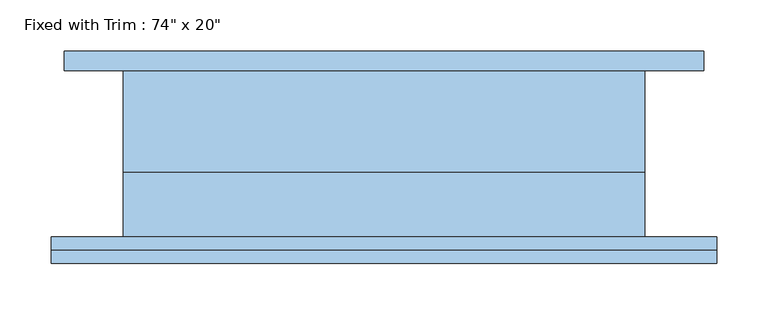
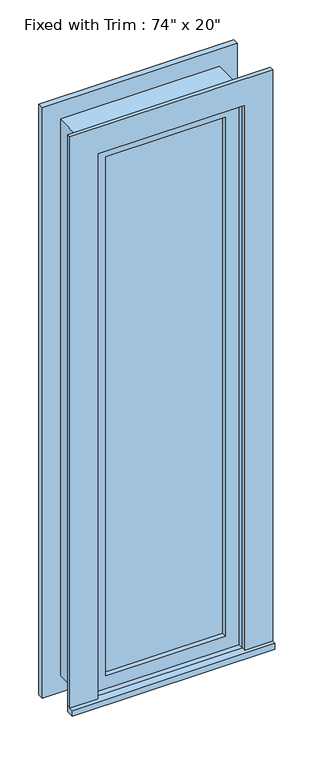
"""IFC4 building model written with IfcOpenShell, lengths in millimetres: window geometry."""

from ifc_helpers import new_model, si_unit, frame, origin, place, context, project, spatial, polyline, outline, extrude, source, transform, mapped, element, save


def window_f2480f1b(model_context):
    return source(origin(), model_context, "Body", "SweptSolid", [
        extrude(outline(polyline([(-361.95, -106.3625), (-361.95, -80.9625), (285.75, -80.9625), (285.75, -106.3625), (-361.95, -106.3625)])), frame((0.0, 0.0, 914.4), z_axis=(0.0, 0.0, 1.0), x_axis=(1.0, 0.0, 0.0)), (0.0, 0.0, 1.0), 19.05),
        extrude(outline(polyline([(2774.95, -273.05), (2774.95, 196.85), (933.45, 196.85), (933.45, 285.75), (2863.85, 285.75), (2863.85, -361.95), (933.45, -361.95), (933.45, -273.05), (2774.95, -273.05)])), frame((0.0, -93.6625, 0.0), z_axis=(0.0, 1.0, 0.0), x_axis=(0.0, 0.0, 1.0)), (0.0, 0.0, 1.0), 12.7),
        extrude(outline(polyline([(2851.15, 273.05), (2851.15, -349.25), (857.25, -349.25), (857.25, 273.05), (2851.15, 273.05)]), holes=[polyline([(2762.25, 184.15), (946.15, 184.15), (946.15, -260.35), (2762.25, -260.35), (2762.25, 184.15)])]), frame((0.0, 80.9625, 0.0), z_axis=(0.0, 1.0, 0.0), x_axis=(0.0, 0.0, 1.0)), (0.0, 0.0, 1.0), 19.05),
        extrude(outline(polyline([(152.4, -33.3375), (152.4, -46.0375), (-228.6, -46.0375), (-228.6, -33.3375), (152.4, -33.3375)])), frame((0.0, 0.0, 977.9), z_axis=(0.0, 0.0, 1.0), x_axis=(1.0, 0.0, 0.0)), (0.0, 0.0, 1.0), 1752.6),
        extrude(outline(polyline([(2774.95, -273.05), (933.45, -273.05), (933.45, 196.85), (2774.95, 196.85), (2774.95, -273.05)]), holes=[polyline([(2730.5, -228.6), (2730.5, 152.4), (977.9, 152.4), (977.9, -228.6), (2730.5, -228.6)])]), frame((0.0, -61.9125, 0.0), z_axis=(0.0, 1.0, 0.0), x_axis=(0.0, 0.0, 1.0)), (0.0, 0.0, 1.0), 44.45),
        extrude(outline(polyline([(2794.0, -292.1), (914.4, -292.1), (914.4, 215.9), (2794.0, 215.9), (2794.0, -292.1)]), holes=[polyline([(2762.25, -260.35), (2762.25, 184.15), (946.15, 184.15), (946.15, -260.35), (2762.25, -260.35)])]), frame((0.0, -17.4625, 0.0), z_axis=(0.0, 1.0, 0.0), x_axis=(0.0, 0.0, 1.0)), (0.0, 0.0, 1.0), 98.425),
        extrude(outline(polyline([(2794.0, 215.9), (2794.0, -292.1), (914.4, -292.1), (914.4, 215.9), (2794.0, 215.9)]), holes=[polyline([(2774.95, 196.85), (933.45, 196.85), (933.45, -273.05), (2774.95, -273.05), (2774.95, 196.85)])]), frame((0.0, -80.9625, 0.0), z_axis=(0.0, 1.0, 0.0), x_axis=(0.0, 0.0, 1.0)), (0.0, 0.0, 1.0), 63.5),
    ])


if __name__ == "__main__":
    model = new_model("IFC4")
    model_context = context("Model", 3, world=origin())
    ifc_project = project(units=[si_unit("LENGTHUNIT", "METRE", prefix="MILLI")], contexts=[model_context])
    site = spatial("IfcSite", under=ifc_project)
    building = spatial("IfcBuilding", under=site)
    placement = place(None, origin())
    window_shape = window_f2480f1b(model_context)
    element("IfcWindow", 1, ObjectType="Fixed with Trim : 74\" x 20\"", at=placement, inside=building, context=model_context, shape_type="MappedRepresentation", body=[
        mapped(window_shape, transform((0.0, 0.0, 0.0), x_axis=(1.0, 0.0, 0.0), y_axis=(0.0, 1.0, 0.0), z_axis=(0.0, 0.0, 1.0))),
    ])
    save(model, "model.ifc")

# Revit data of these elements
# Type "Fixed with Trim : 74\" x 20\""
#   Type Mark = "59"
#   COBie.Type.CreatedBy = "doug.wood@us.ibm.com"
#   COBie.Type.CreatedOn = "2016-04-14T02:07:26"
#   COBie.Type.Name = "Windows_Fixed with Trim_74\" x 20\"_59"
#   COBie.Type.Category = "23-30 20 17 11 : Fixed Windows"
#   COBie.Type.Description = "Fixed with Trim_74\" x 20\""
#   COBie.Type.Manufacturer = ""
#   COBie.Type.ModelNumber = ""
#   Construction Type Id = "GSP4R"
#   Assembly Code = "B2020100"
#   Analytic Construction = "1/8 in Pilkington single glazing"
#   COBie.Type.ReplacementCost = 0
#   Visual Light Transmittance = 0.9
#   Solar Heat Gain Coefficient = 0.78
#   Heat Transfer Coefficient (U) = 3.6886 W/(m²·K)
#   Height = 6' - 2"
#   Default Sill Height = 3' - 0"
#   Trim Projection - Ext. = 0' - 0 1/2"
#   Trim Projection - Int. = 0' - 0 3/4"
#   Trim Width - Exterior = 0' - 3 1/2"
#   Trim Width - Interior = 0' - 3 1/2"
#   Width = 1' - 8"
#   Window Inset = 0' - 0 3/4"
#   COBie.Type = no
#   Glass Pane Material = Glass
#   Sash Material = Sash - White
#   Trim Exterior Material = Trim - White
#   Trim Interior Material = Trim - White
#   Wall Closure = (empty or 0)
# Element 1 (IfcWindow, "Fixed with Trim : 74\" x 20\"")
#   Materials on its faces: "Sash - White", "Trim - White", "Glass"
# Materials
#   "Glass": class "Glass", colour RGB 0 128 192, transparency 0.75, Description = "Soda Lime Glass", Cost = 0
#   "Sash - White": class "Wood", colour RGB 255 255 255, transparency 0, Cost = 0
#   "Trim - White": class "Wood", colour RGB 255 255 255, transparency 0, Cost = 0
